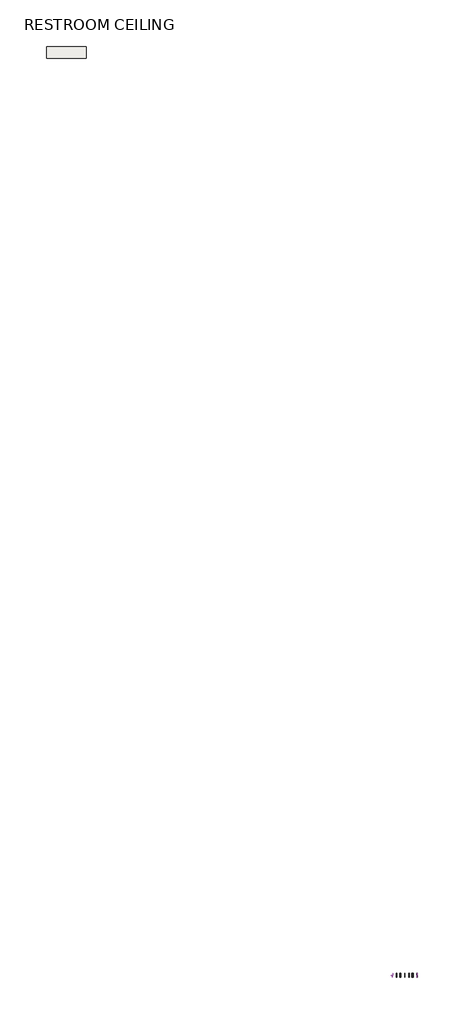
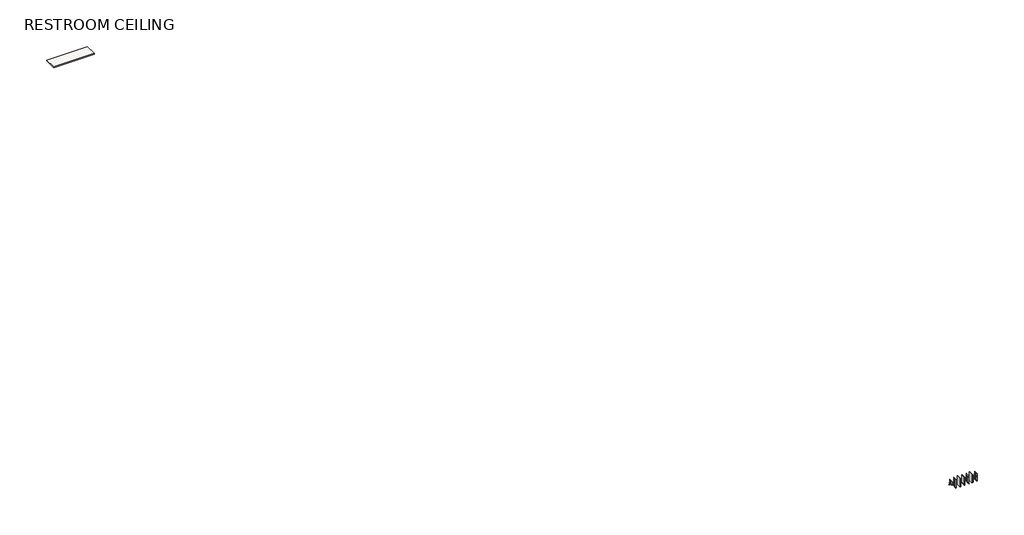
# One storey: 61 proxies, 1 slab.
# Revit data of these elements (continued)
# Element 30 (IfcBuildingElementProxy, "Generic Models 246 : Generic Models 1")
#   Phase Created = _ZAVE_2
#   Materials on its faces: "BULKHEAD FRAME WORK"
# Element 31 (IfcBuildingElementProxy, "Generic Models 248 : Generic Models 65")
#   Phase Created = _ZAVE_2
#   Materials on its faces: "2X WOOD STUD - SEE 'WALL TAG' & 'LAYER MATERIAL SCHEDULE' FOR SPACING & INSULATION TREATMENT, IF APPLICAPLE"
# Element 32 (IfcBuildingElementProxy, "Generic Models 249 : Generic Models 1")
#   Phase Created = _ZAVE_2
#   Materials on its faces: "ACOUSTICAL SEALANT"
# Element 33 (IfcBuildingElementProxy, "Generic Models 253 : Generic Models 1")
#   Phase Created = _ZAVE_2
#   Materials on its faces: "MATCH EXISTING BASE"
# Element 34 (IfcBuildingElementProxy, "Generic Models 260 : Generic Models 1")
#   Phase Created = _ZAVE_2
#   Materials on its faces: "(S) SOUND BATT. INSULATION (THICKNESS TO MATCH WALL DEPTH)"
# Element 35 (IfcBuildingElementProxy, "Generic Models 262 : Generic Models 65")
#   Phase Created = _ZAVE_2
#   Materials on its faces: "2X WOOD STUD - SEE 'WALL TAG' & 'LAYER MATERIAL SCHEDULE' FOR SPACING & INSULATION TREATMENT, IF APPLICAPLE"
# Element 36 (IfcBuildingElementProxy, "Generic Models 268 : Generic Models 46")
#   Phase Created = _ZAVE_2
#   Materials on its faces: "6 MIL VAPOR BARRIER"
# Element 37 (IfcBuildingElementProxy, "Generic Models 3 : Generic Models 1")
#   Phase Created = _ZAVE_2
#   Materials on its faces: "ACOUSTICAL SEALANT"
# Element 38 (IfcBuildingElementProxy, "Generic Models 40 : Generic Models 1")
#   Phase Created = _ZAVE_2
#   Materials on its faces: "TREATED 2X WOOD SILL"
# Element 39 (IfcBuildingElementProxy, "Generic Models 41 : Generic Models 1")
#   Phase Created = _ZAVE_2
#   Materials on its faces: "ACOUSTICAL SEALANT"
# Element 40 (IfcBuildingElementProxy, "Generic Models 42 : Generic Models 1")
#   Phase Created = _ZAVE_2
#   Materials on its faces: "MATCH EXISTING BASE"
# Element 41 (IfcBuildingElementProxy, "Generic Models 44 : Generic Models 1")
#   Phase Created = _ZAVE_2
#   Materials on its faces: "5/8\" GYP. BD"
# Element 42 (IfcBuildingElementProxy, "Generic Models 45 : Generic Models 1")
#   Phase Created = _ZAVE_2
#   Materials on its faces: "ACOUSTICAL SEALANT"
# Element 43 (IfcBuildingElementProxy, "Generic Models 5 : Generic Models 1")
#   Phase Created = _ZAVE_2
#   Materials on its faces: "MATCH EXISTING BASE"
# Element 44 (IfcBuildingElementProxy, "Generic Models 50 : Generic Models 1")
#   Phase Created = _ZAVE_2
#   Materials on its faces: "MATCH EXISTING BASE"
# Element 45 (IfcBuildingElementProxy, "Generic Models 52 : Generic Models 65")
#   Phase Created = _ZAVE_2
#   Materials on its faces: "2X WOOD STUD - SEE 'WALL TAG' & 'LAYER MATERIAL SCHEDULE' FOR SPACING & INSULATION TREATMENT, IF APPLICAPLE"
# Element 46 (IfcBuildingElementProxy, "Generic Models 55 : Generic Models 1")
#   Phase Created = _ZAVE_2
#   Materials on its faces: "5/8\" GYP. BD"
# Element 47 (IfcBuildingElementProxy, "Generic Models 56 : Generic Models 1")
#   Phase Created = _ZAVE_2
#   Materials on its faces: "TREATED 2X WOOD SILL"
# Element 48 (IfcBuildingElementProxy, "Generic Models 57 : Generic Models 1")
#   Phase Created = _ZAVE_2
#   Materials on its faces: "ACOUSTICAL SEALANT"
# Element 49 (IfcBuildingElementProxy, "Generic Models 58 : Generic Models 1")
#   Phase Created = _ZAVE_2
#   Materials on its faces: "MATCH EXISTING BASE"
# Element 50 (IfcBuildingElementProxy, "Generic Models 60 : Generic Models 1")
#   Phase Created = _ZAVE_2
#   Materials on its faces: "5/8\" GYP. BD"
# Element 51 (IfcBuildingElementProxy, "Generic Models 63 : Generic Models 1")
#   Phase Created = _ZAVE_2
#   Materials on its faces: "(S) SOUND BATT. INSULATION (THICKNESS TO MATCH WALL DEPTH)"
# Element 52 (IfcBuildingElementProxy, "Generic Models 65 : Generic Models 65")
#   Phase Created = _ZAVE_2
#   Materials on its faces: "2X WOOD STUD - SEE 'WALL TAG' & 'LAYER MATERIAL SCHEDULE' FOR SPACING & INSULATION TREATMENT, IF APPLICAPLE"
# Element 53 (IfcBuildingElementProxy, "Generic Models 68 : Generic Models 1")
#   Phase Created = _ZAVE_2
#   Materials on its faces: "ACOUSTICAL SEALANT"
# Element 54 (IfcBuildingElementProxy, "Generic Models 69 : Generic Models 1")
#   Phase Created = _ZAVE_2
#   Materials on its faces: "5/8\" GYP. BD"
# Element 55 (IfcBuildingElementProxy, "Generic Models 7 : Generic Models 1")
#   Phase Created = _ZAVE_2
#   Materials on its faces: "(S) SOUND BATT. INSULATION (THICKNESS TO MATCH WALL DEPTH)"
# Element 56 (IfcBuildingElementProxy, "Generic Models 73 : Generic Models 1")
#   Phase Created = _ZAVE_2
#   Materials on its faces: "MATCH EXISTING BASE"
# Element 57 (IfcBuildingElementProxy, "Generic Models 76 : Generic Models 1")
#   Phase Created = _ZAVE_2
#   Materials on its faces: "CMU (SEE 'WALL TAGE' FOR SIZE)"
# Element 58 (IfcBuildingElementProxy, "Generic Models 85 : Generic Models 65")
#   Phase Created = _ZAVE_2
#   Materials on its faces: "2X WOOD STUD - SEE 'WALL TAG' & 'LAYER MATERIAL SCHEDULE' FOR SPACING & INSULATION TREATMENT, IF APPLICAPLE"
# Element 59 (IfcBuildingElementProxy, "Generic Models 9 : Generic Models 1")
#   Phase Created = _ZAVE_2
#   Materials on its faces: "GYP. BD (SEE 'WALL TAG' & 'LAYER MATERIAL SCHEDULE' FOR DETAILS)"
# Element 60 (IfcBuildingElementProxy, "Generic Models 90 : Generic Models 1")
#   Phase Created = _ZAVE_2
#   Materials on its faces: "ACOUSTICAL SEALANT"
# Element 61 (IfcBuildingElementProxy, "Generic Models 92 : Generic Models 1")
#   Phase Created = _ZAVE_2
#   Materials on its faces: "MATCH EXISTING BASE"
# Element 62 (IfcSlab, "RESTROOMS CEILING")
#   Height Offset From Level = 0' - 0"
#   Phase Created = 1st Phase
#   Materials on its faces: "5/8\" GYP. BD", "3/4\" CDX PLYWOOD"
# Materials
#   "3/4\" CDX PLYWOOD": class "Unassigned", colour RGB 196 177 123, transparency 0, Cost = 0
#   "9 1/2\" TJI JOISTS": class "Wood", colour RGB 234 198 147, transparency 0, Description = "Pinus Echinata", Cost = 0
#   "5/8\" GYP. BD": class "Generic", colour RGB 255 255 255, transparency 0, Description = "Gypsum Wall Board", Cost = 0
#   "TREATED 2X WOOD SILL": class "Wood", colour RGB 234 198 147, transparency 0, Description = "Pinus Echinata", Cost = 0
#   "(S) SOUND BATT. INSULATION (THICKNESS TO MATCH WALL DEPTH)": class "Unassigned", colour RGB 255 255 255, transparency 0, Cost = 0
#   "2X WOOD STUD - SEE 'WALL TAG' & 'LAYER MATERIAL SCHEDULE' FOR SPACING & INSULATION TREATMENT, IF APPLICAPLE": class "Wood", colour RGB 234 198 147, transparency 0, Description = "Pinus Echinata", Cost = 0
#   "EXISTING GIRT": class "Metal", colour RGB 199 199 199, transparency 0, Description = "Carbon steel", Cost = 0
#   "2X WOOD HEADER ATTACHED TO EXISTING JOIST": class "Wood", colour RGB 234 198 147, transparency 0, Description = "Pinus Echinata", Cost = 0
#   "WOOD BLOCKING - SIZE AS NECESSARY": class "Wood", colour RGB 234 198 147, transparency 0, Description = "Pinus Echinata", Cost = 0
#   "GYP. BD (SEE 'WALL TAG' & 'LAYER MATERIAL SCHEDULE' FOR DETAILS)": class "Generic", colour RGB 237 236 233, transparency 0, Description = "Gypsum Wall Board", Cost = 0
#   "ACOUSTICAL SEALANT": class "Unassigned", colour RGB 120 120 120, transparency 0, Cost = 0
#   "MATCH EXISTING BASE": class "Generic", colour RGB 120 120 120, transparency 0, Cost = 0
#   "6 MIL VAPOR BARRIER": class "Generic", colour RGB 66 158 52, transparency 0, Cost = 0
#   "BULKHEAD FRAME WORK": class "Metal", colour RGB 189 187 185, transparency 0, Description = "Structural steel 50ksi", Cost = 0
#   "EXISTING WALL": class "Generic", colour RGB 201 201 201, transparency 0, Cost = 0
#   "CMU (SEE 'WALL TAGE' FOR SIZE)": class "Masonry", colour RGB 203 203 199, transparency 0, Description = "Concrete masonry units", Cost = 0
